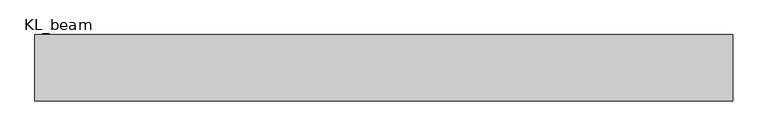
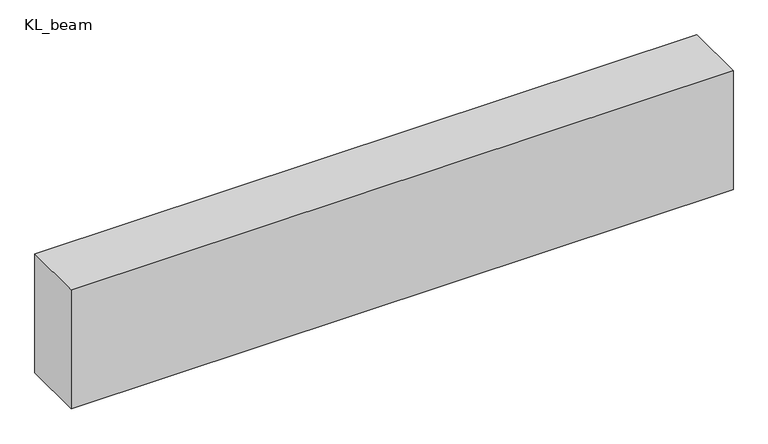
"""IFC4 building model written with IfcOpenShell, lengths in millimetres: beam geometry, 混凝土 - 矩形梁 : KL_beam."""

from ifc_helpers import new_model, si_unit, frame, origin, place, context, project, spatial, polyline, outline, extrude, source, transform, mapped, element, save


def kl_beam_b765c5bf(model_context):
    return source(origin(), model_context, "Body", "SweptSolid", [
        extrude(outline(polyline([(2105.0, 200.0), (2105.0, -200.0), (-2105.0, -200.0), (-2105.0, 200.0), (2105.0, 200.0)])), frame((0.0, 0.0, -400.0), z_axis=(0.0, 0.0, 1.0), x_axis=(1.0, 0.0, 0.0)), (0.0, 0.0, 1.0), 800.0),
    ])


if __name__ == "__main__":
    model = new_model("IFC4")
    model_context = context("Model", 3, world=origin())
    ifc_project = project(units=[si_unit("LENGTHUNIT", "METRE", prefix="MILLI")], contexts=[model_context])
    site = spatial("IfcSite", under=ifc_project)
    building = spatial("IfcBuilding", under=site)
    placement = place(None, origin())
    kl_beam_shape = kl_beam_b765c5bf(model_context)
    element("IfcBeam", 1, ObjectType="混凝土 - 矩形梁 : KL_beam", at=placement, inside=building, context=model_context, shape_type="MappedRepresentation", body=[
        mapped(kl_beam_shape, transform((0.0, 0.0, 0.0), x_axis=(1.0, 0.0, 0.0), y_axis=(0.0, 1.0, 0.0), z_axis=(0.0, 0.0, 1.0))),
    ])
    save(model, "model.ifc")

# Revit data of these elements
# Type "混凝土 - 矩形梁 : KL_beam"
#   Length [instance default] = 1524 mm
#   b = 400 mm
#   h = 800 mm
#   Structural Material [instance default] = 混凝土 - 现场浇注混凝土
#   Assembly Code = ""
# Element 1 (IfcBeam, "混凝土 - 矩形梁 : KL_beam")
#   Structural Material = none
# Materials
#   "混凝土 - 现场浇注混凝土": class "混凝土", colour RGB 192 192 192, transparency 0
